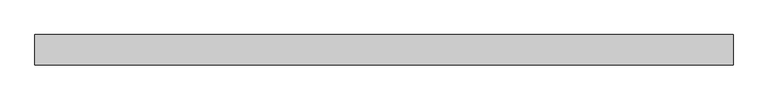
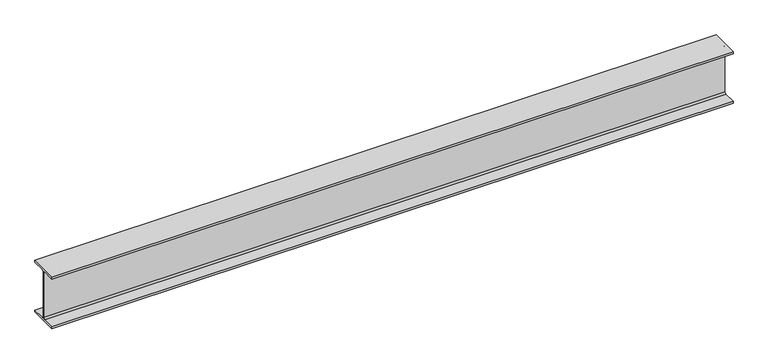
"""IFC4 building model written with IfcOpenShell, lengths in millimetres: beam geometry, Old_Steel Beam_H-KSD3502 : H_SB_ASB_H-250×125x6x9."""

from ifc_helpers import new_model, si_unit, point, frame, frame_2d, origin, place, context, project, spatial, polyline, circle_curve, trimmed, segment, composite_curve, outline, extrude, source, transform, mapped, element, save


def beam_8ddbad79(model_context):
    return source(origin(), model_context, "Body", "SweptSolid", [
        extrude(outline(composite_curve([segment(polyline([(82.5, -141.5), (82.5, -151.7), (-82.5, -151.7), (-82.5, -141.5), (-11.9, -141.5)]), True, "CONTINUOUS"), segment(trimmed(circle_curve(frame_2d((-11.9, -132.6)), 8.9), [point((-11.9, -141.5))], [point((-3.0, -132.6))], True, "CARTESIAN"), True, "CONTINUOUS"), segment(polyline([(-3.0, -132.6), (-3.0, 132.6)]), True, "CONTINUOUS"), segment(trimmed(circle_curve(frame_2d((-11.9, 132.6)), 8.9), [point((-3.0, 132.6))], [point((-11.9, 141.5))], True, "CARTESIAN"), True, "CONTINUOUS"), segment(polyline([(-11.9, 141.5), (-82.5, 141.5), (-82.5, 151.7), (82.5, 151.7), (82.5, 141.5), (11.9, 141.5)]), True, "CONTINUOUS"), segment(trimmed(circle_curve(frame_2d((11.9, 132.6)), 8.9), [point((11.9, 141.5))], [point((3.0, 132.6))], True, "CARTESIAN"), True, "CONTINUOUS"), segment(polyline([(3.0, 132.6), (3.0, -132.6)]), True, "CONTINUOUS"), segment(trimmed(circle_curve(frame_2d((11.9, -132.6)), 8.9), [point((3.0, -132.6))], [point((11.9, -141.5))], True, "CARTESIAN"), True, "CONTINUOUS"), segment(polyline([(11.9, -141.5), (82.5, -141.5)]), True, "CONTINUOUS")], self_intersect=False)), frame((-1904.8, 0.0, 0.0), z_axis=(1.0, 0.0, 0.0), x_axis=(0.0, 1.0, 0.0)), (0.0, 0.0, 1.0), 3809.6),
    ])


if __name__ == "__main__":
    model = new_model("IFC4")
    model_context = context("Model", 3, world=origin())
    ifc_project = project(units=[si_unit("LENGTHUNIT", "METRE", prefix="MILLI")], contexts=[model_context])
    site = spatial("IfcSite", under=ifc_project)
    building = spatial("IfcBuilding", under=site)
    placement = place(None, origin())
    beam_shape = beam_8ddbad79(model_context)
    element("IfcBeam", 1, ObjectType="Old_Steel Beam_H-KSD3502 : H_SB_ASB_H-250×125x6x9", at=placement, inside=building, context=model_context, shape_type="MappedRepresentation", body=[
        mapped(beam_shape, transform((0.0, 0.0, 0.0), x_axis=(1.0, 0.0, 0.0), y_axis=(0.0, 1.0, 0.0), z_axis=(0.0, 0.0, 1.0))),
    ])
    save(model, "model.ifc")

# Revit data of these elements
# Type "Old_Steel Beam_H-KSD3502 : H_SB_ASB_H-250×125x6x9"
#   Width = 12.5 cm
#   Web Thickness = 0.6 cm
#   Web Fillet = 1.2 cm
#   Warping Constant = 42539.8 cm⁶
#   Torsional Moment of Inertia = 7.8102 cm⁴
#   Torsional Modulus = 1.0 cm³
#   Section Area = 37.66 cm²
#   Plastic Modulus weak axis = 73.1 cm³
#   Plastic Modulus strong axis = 366.0 cm³
#   Perimeter = 0.97 m²/m
#   Nominal Weight = 29.60 kgf/m
#   Moment of Inertia weak axis = 294.00 cm⁴
#   Moment of Inertia strong axis = 4050.00 cm⁴
#   Height = 25.0 cm
#   Flange Thickness = 0.9 cm
#   Elastic Modulus weak axis = 47.0 cm³
#   Elastic Modulus strong axis = 324.0 cm³
#   Centroid Vertical = 12.5 cm
#   Centroid Horizontal = 6.25 cm
#   Length [instance default] = 1.5240 m
#   Structural Material [instance default] = Steel, 45-345
#   Assembly Code = ""
# Element 1 (IfcBeam, "Old_Steel Beam_H-KSD3502 : H_SB_ASB_H-250×125x6x9")
#   Structural Material = none
# Materials
#   "Steel, 45-345": class "Metal", colour RGB 189 187 185, transparency 0, Description = "Steel 345 MPa", Cost = 0
